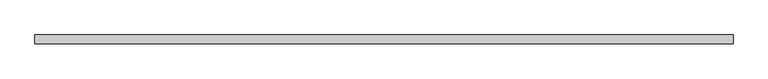
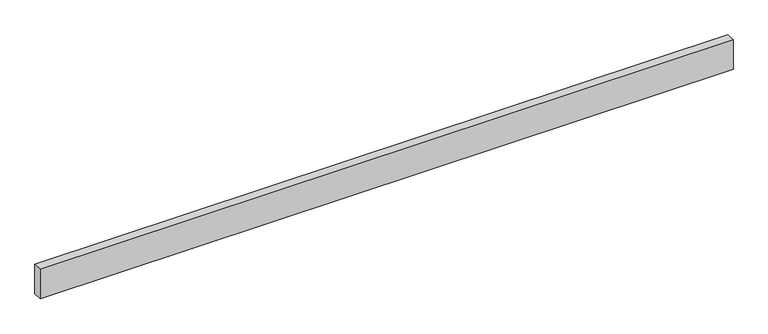
"""IFC4 building model written with IfcOpenShell, lengths in millimetres: beam geometry, NLRS_28_SF_LIB_houten balk-MMBW-SRP_gen_rsf : houten balk_gen__bxh 70x195."""

from ifc_helpers import new_model, si_unit, frame, origin, place, context, project, spatial, polyline, outline, extrude, source, transform, mapped, element, save


def beam_9365c9be(model_context):
    return source(origin(), model_context, "Body", "SweptSolid", [
        extrude(outline(polyline([(-2751.0, -35.0), (-2751.0, 35.0), (2751.0, 35.0), (2751.0, -35.0), (-2751.0, -35.0)])), frame((0.0, 0.0, -122.5), z_axis=(0.0, 0.0, 1.0), x_axis=(1.0, 0.0, 0.0)), (0.0, 0.0, 1.0), 245.0),
    ])


if __name__ == "__main__":
    model = new_model("IFC4")
    model_context = context("Model", 3, world=origin())
    ifc_project = project(units=[si_unit("LENGTHUNIT", "METRE", prefix="MILLI")], contexts=[model_context])
    site = spatial("IfcSite", under=ifc_project)
    building = spatial("IfcBuilding", under=site)
    placement = place(None, origin())
    beam_shape = beam_9365c9be(model_context)
    element("IfcBeam", 1, ObjectType="NLRS_28_SF_LIB_houten balk-MMBW-SRP_gen_rsf : houten balk_gen__bxh 70x195", at=placement, inside=building, context=model_context, shape_type="MappedRepresentation", body=[
        mapped(beam_shape, transform((0.0, 0.0, 0.0), x_axis=(1.0, 0.0, 0.0), y_axis=(0.0, 1.0, 0.0), z_axis=(0.0, 0.0, 1.0))),
    ])
    save(model, "model.ifc")

# Revit data of these elements
# Type "NLRS_28_SF_LIB_houten balk-MMBW-SRP_gen_rsf : houten balk_gen__bxh 70x195"
#   Export Type to IFC As = "IfcBeamType"
#   Type IfcGUID = "07M7mRoiH1CR8m_RSKIvYS"
#   Type Comments = "70x195"
#   Model = " "
#   Manufacturer = " "
#   Fire Rating = " "
#   Description = "houten balk 70x195"
#   Assembly Code = "28.11"
#   NLRS_C_lengte [instance default] = 3000 mm
#   NLRS_C_hoogte = 245 mm
#   NLRS_C_breedte = 70 mm
#   Length [instance default] = 3000 mm
#   Structural Material = NLRS_i2_hout naaldhout vuren_gen_rsf
#   Keynote = ""
# Element 1 (IfcBeam, "NLRS_28_SF_LIB_houten balk-MMBW-SRP_gen_rsf : houten balk_gen__bxh 70x195")
#   NLRS_C_lengte = 5572 mm
#   Materials on its faces: "NLRS_i2_hout naaldhout vuren_gen_rsf"
# Materials
#   "NLRS_i2_hout naaldhout vuren_gen_rsf": class "I - Hout", colour RGB 234 199 147, transparency 0, Keynote = "i2", Manufacturer = "Revit Standards Foundation", URL = "www.revitstandards.org", Description = "hout vuren", Cost = 0
